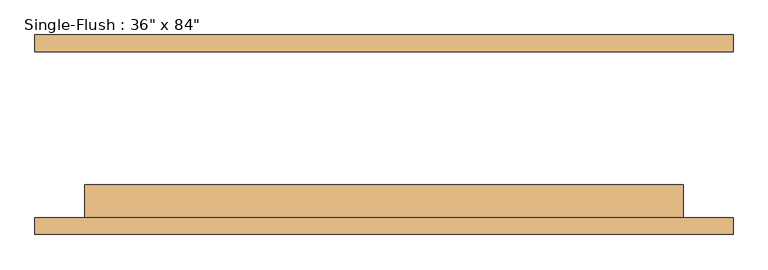
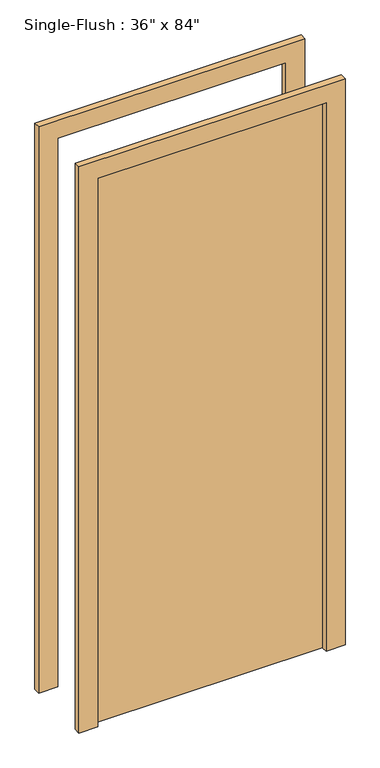
"""IFC4 building model written with IfcOpenShell, lengths in millimetres: door geometry."""

import ifcopenshell
import ifcopenshell.guid

model = None  # the IFC model being written
_history = None  # IfcOwnerHistory: only IFC2X3 demands one
_inside = {}  # id of a spatial element -> (the spatial element, [elements in it])
_under = {}  # id of a project, library or spatial element -> (it, [spatial elements below it])
_declared = {}  # id of a project -> (the project, [libraries it declares])
_typed = {}  # id of a type object -> (the type object, [elements of that type])
_made_of = {}  # id of a material, layer set ... -> (it, [elements and type objects made of it])


def new_model(schema):
    """Start an empty IFC model of exactly this schema.

    Asked for "IFC4X3", IfcOpenShell would pick the latest addendum, in which some entities
    have other attributes; the version numbers below select the first issue.
    IFC2X3 requires an IfcOwnerHistory on every rooted entity: one is made here for all.
    """
    global model, _history
    if schema == "IFC4X3":
        model = ifcopenshell.file(schema_version=(4, 3, 0, 0))
    else:
        model = ifcopenshell.file(schema=schema)
    _inside.clear()
    _under.clear()
    _declared.clear()
    _typed.clear()
    _made_of.clear()
    _history = None
    if model.schema == "IFC2X3":
        org = make("IfcOrganization", Name="unknown")
        user = make(
            "IfcPersonAndOrganization",
            ThePerson=make("IfcPerson", FamilyName="unknown"),
            TheOrganization=org,
        )
        app = make(
            "IfcApplication",
            ApplicationDeveloper=org,
            Version="unknown",
            ApplicationFullName="unknown",
            ApplicationIdentifier="unknown",
        )
        _history = make(
            "IfcOwnerHistory",
            OwningUser=user,
            OwningApplication=app,
            ChangeAction="ADDED",
            CreationDate=0,
        )
    return model


def make(cls, **values):
    """One entity of the class cls with the attributes given. An attribute that is None is left unset."""
    return model.create_entity(
        cls, **{name: value for name, value in values.items() if value is not None}
    )


def rooted(cls, **values):
    """An entity with a GlobalId (a new one), such as an element, a storey or a relation."""
    return make(cls, GlobalId=ifcopenshell.guid.new(), OwnerHistory=_history, **values)


def si_unit(unit_type, name, prefix=None):
    """IfcSIUnit, for example si_unit("LENGTHUNIT", "METRE", prefix="MILLI")."""
    return make("IfcSIUnit", UnitType=unit_type, Prefix=prefix, Name=name)


def assignment(units):
    """IfcUnitAssignment: the units of a project."""
    return None if units is None else make("IfcUnitAssignment", Units=units)


def point(xyz):
    """IfcCartesianPoint."""
    return None if xyz is None else make("IfcCartesianPoint", Coordinates=xyz)


def direction(xyz):
    """IfcDirection."""
    return None if xyz is None else make("IfcDirection", DirectionRatios=xyz)


def frame(location, z_axis=None, x_axis=None):
    """IfcAxis2Placement3D, a coordinate frame: its origin and axes. An axis left out is left unset."""
    return make(
        "IfcAxis2Placement3D",
        Location=point(location),
        Axis=direction(z_axis),
        RefDirection=direction(x_axis),
    )


def origin():
    """The frame at (0, 0, 0) with its axes left unset."""
    return frame((0.0, 0.0, 0.0))


def origin_with_axes():
    """The frame at (0, 0, 0) with the z axis (0, 0, 1) and the x axis (1, 0, 0) written out."""
    return frame((0.0, 0.0, 0.0), z_axis=(0.0, 0.0, 1.0), x_axis=(1.0, 0.0, 0.0))


def place(relative_to, where):
    """IfcLocalPlacement: puts the frame where relative to a parent placement (None: the world)."""
    return make(
        "IfcLocalPlacement", PlacementRelTo=relative_to, RelativePlacement=where
    )


def context(
    kind, dimensions, precision=None, world=None, true_north=None, identifier=None
):
    """IfcGeometricRepresentationContext, for example the 3D "Model" context."""
    return make(
        "IfcGeometricRepresentationContext",
        ContextIdentifier=identifier,
        ContextType=kind,
        CoordinateSpaceDimension=dimensions,
        Precision=precision,
        WorldCoordinateSystem=world,
        TrueNorth=true_north,
    )


def project(units=None, contexts=None):
    """IfcProject with its units and contexts."""
    return rooted(
        "IfcProject",
        Name="project",
        RepresentationContexts=contexts,
        UnitsInContext=assignment(units),
    )


def spatial(cls, under=None, at=None, **own):
    """A site, building, storey or space (cls), placed at a placement, below another one or the project."""
    s = rooted(cls, ObjectPlacement=at, **own)
    if under is not None:
        _under.setdefault(under.id(), (under, []))[1].append(s)
    return s


def polyline(points):
    """IfcPolyline through the points."""
    return make("IfcPolyline", Points=[point(p) for p in points])


def outline(outer, holes=None, kind="AREA"):
    """IfcArbitraryClosedProfileDef: a profile drawn as a closed curve; with holes, ...WithVoids."""
    if holes is None:
        return make("IfcArbitraryClosedProfileDef", ProfileType=kind, OuterCurve=outer)
    return make(
        "IfcArbitraryProfileDefWithVoids",
        ProfileType=kind,
        OuterCurve=outer,
        InnerCurves=holes,
    )


def extrude(swept, where, along, depth):
    """IfcExtrudedAreaSolid: the profile swept, set in the frame where, extruded along a direction by depth."""
    return make(
        "IfcExtrudedAreaSolid",
        SweptArea=swept,
        Position=where,
        ExtrudedDirection=direction(along),
        Depth=depth,
    )


def shape(context_of_items, identifier, shape_type, items):
    """IfcShapeRepresentation: the items that make up one representation, for example the "Body"."""
    return make(
        "IfcShapeRepresentation",
        ContextOfItems=context_of_items,
        RepresentationIdentifier=identifier,
        RepresentationType=shape_type,
        Items=items,
    )


def source(mapping_origin, context_of_items, identifier, shape_type, items):
    """IfcRepresentationMap: a shape defined once, which mapped items show again and again."""
    return make(
        "IfcRepresentationMap",
        MappingOrigin=mapping_origin,
        MappedRepresentation=shape(context_of_items, identifier, shape_type, items),
    )


def transform(
    local_origin,
    x_axis=None,
    y_axis=None,
    z_axis=None,
    scale=None,
    scale2=None,
    scale3=None,
    uniform=True,
):
    """IfcCartesianTransformationOperator3D, or its non-uniform kind. x_axis, y_axis, z_axis: its Axis1, 2, 3."""
    if uniform:
        return make(
            "IfcCartesianTransformationOperator3D",
            Axis1=direction(x_axis),
            Axis2=direction(y_axis),
            LocalOrigin=point(local_origin),
            Scale=scale,
            Axis3=direction(z_axis),
        )
    return make(
        "IfcCartesianTransformationOperator3DnonUniform",
        Axis1=direction(x_axis),
        Axis2=direction(y_axis),
        LocalOrigin=point(local_origin),
        Scale=scale,
        Axis3=direction(z_axis),
        Scale2=scale2,
        Scale3=scale3,
    )


def mapped(mapping_source, mapping_target):
    """IfcMappedItem: shows the shape of a source again, moved by a transform."""
    return make(
        "IfcMappedItem", MappingSource=mapping_source, MappingTarget=mapping_target
    )


def made_of(thing, what):
    """Note that an element or type object is made of a material, layer set ...; save() writes the relation."""
    if what is not None:
        _made_of.setdefault(what.id(), (what, []))[1].append(thing)
    return thing


def element(
    cls,
    number,
    at=None,
    inside=None,
    cuts=None,
    type_object=None,
    material=None,
    context=None,
    identifier="Body",
    shape_type=None,
    held_by="IfcProductDefinitionShape",
    body=None,
    shapes=None,
    **own,
):
    """One element of the class cls, such as IfcWall. Its Tag is "e" and its number.

    at: its placement. inside: the storey or other place that contains it. cuts: it is an
    opening in that element (IfcRelVoidsElement). A single representation is given by context,
    identifier, shape_type and body (its items); several are given by shapes. held_by: the class
    of the entity that holds the representations. save() writes the other relations.
    """
    e = rooted(cls, Tag="e%d" % number, ObjectPlacement=at, **own)
    if body is not None:
        shapes = [shape(context, identifier, shape_type, body)]
    if shapes is not None:
        e.Representation = make(held_by, Representations=shapes)
    if inside is not None:
        _inside.setdefault(inside.id(), (inside, []))[1].append(e)
    if cuts is not None:
        rooted(
            "IfcRelVoidsElement", RelatingBuildingElement=cuts, RelatedOpeningElement=e
        )
    if type_object is not None:
        _typed.setdefault(type_object.id(), (type_object, []))[1].append(e)
    return made_of(e, material)


def aggregate(whole, parts):
    """IfcRelAggregates: a whole, such as a stair, and the parts it consists of."""
    return rooted("IfcRelAggregates", RelatingObject=whole, RelatedObjects=parts)


def save(model, path):
    """Write the relations noted so far, then the file.

    IfcRelAggregates (storeys below a building ...), IfcRelContainedInSpatialStructure (elements
    in a storey), IfcRelDefinesByType, IfcRelAssociatesMaterial and IfcRelDeclares: one each for
    every whole, place, type object, material and project.
    """
    for whole, parts in _under.values():
        aggregate(whole, parts)
    for where, things in _inside.values():
        rooted(
            "IfcRelContainedInSpatialStructure",
            RelatedElements=things,
            RelatingStructure=where,
        )
    for kind, things in _typed.values():
        rooted("IfcRelDefinesByType", RelatedObjects=things, RelatingType=kind)
    for what, things in _made_of.values():
        rooted("IfcRelAssociatesMaterial", RelatedObjects=things, RelatingMaterial=what)
    for by, libraries in _declared.values():
        rooted("IfcRelDeclares", RelatingContext=by, RelatedDefinitions=libraries)
    model.write(path)


def door_90ca7aae(model_context):
    return source(origin(), model_context, "Body", "SweptSolid", [
        extrude(outline(polyline([(2399.6, -533.4), (0.0, -533.4), (0.0, -457.2), (2323.4, -457.2), (2323.4, 457.2), (0.0, 457.2), (0.0, 533.4), (2399.6, 533.4), (2399.6, -533.4)])), frame((0.0, -152.4, 0.0), z_axis=(0.0, 1.0, 0.0), x_axis=(0.0, 0.0, 1.0)), (0.0, 0.0, 1.0), 25.4),
        extrude(outline(polyline([(2399.6, 533.4), (2399.6, -533.4), (0.0, -533.4), (0.0, -457.2), (2323.4, -457.2), (2323.4, 457.2), (0.0, 457.2), (0.0, 533.4), (2399.6, 533.4)])), frame((0.0, 127.0, 0.0), z_axis=(0.0, 1.0, 0.0), x_axis=(0.0, 0.0, 1.0)), (0.0, 0.0, 1.0), 25.4),
        extrude(outline(polyline([(457.2, -76.2), (457.2, -127.0), (-457.2, -127.0), (-457.2, -76.2), (457.2, -76.2)])), origin_with_axes(), (0.0, 0.0, 1.0), 2323.4),
    ])


if __name__ == "__main__":
    model = new_model("IFC4")
    model_context = context("Model", 3, world=origin())
    ifc_project = project(units=[si_unit("LENGTHUNIT", "METRE", prefix="MILLI")], contexts=[model_context])
    site = spatial("IfcSite", under=ifc_project)
    building = spatial("IfcBuilding", under=site)
    placement = place(None, origin())
    door_shape = door_90ca7aae(model_context)
    element("IfcDoor", 1, ObjectType="Single-Flush : 36\" x 84\"", at=placement, inside=building, context=model_context, shape_type="MappedRepresentation", body=[
        mapped(door_shape, transform((0.0, 0.0, 0.0), x_axis=(1.0, 0.0, 0.0), y_axis=(0.0, 1.0, 0.0), z_axis=(0.0, 0.0, 1.0))),
    ])
    save(model, "model.ifc")

# Revit data of these elements
# Type "Single-Flush : 36\" x 84\""
#   Type Mark = "D2"
#   Construction Type Id = "MDOOR"
#   Assembly Code = "C1020"
#   Analytic Construction = "Metal"
#   Thickness = 50.8 mm
#   Heat Transfer Coefficient (U) = 3.7021 W/(m²·K)
#   Height = 2323.4 mm
#   Trim Projection Ext = 25.4 mm
#   Trim Projection Int = 25.4 mm
#   Trim Width = 76.2 mm
#   Width = 914.4 mm
#   Define Thermal Properties by = 1
#   Door Material = wooden-3
#   Frame Material = wooden-3
#   Visual Light Transmittance = 0
#   Solar Heat Gain Coefficient = 0
#   Function = (empty or 0)
#   Wall Closure = (empty or 0)
# Element 1 (IfcDoor, "Single-Flush : 36\" x 84\"")
#   Materials on its faces: "wooden-3"
# Materials
#   "wooden-3": class "Generic", colour RGB 120 120 120, transparency 0, Cost = 0
